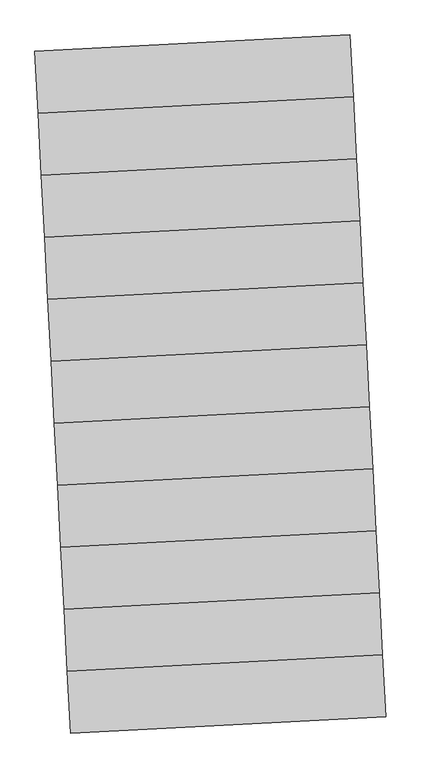
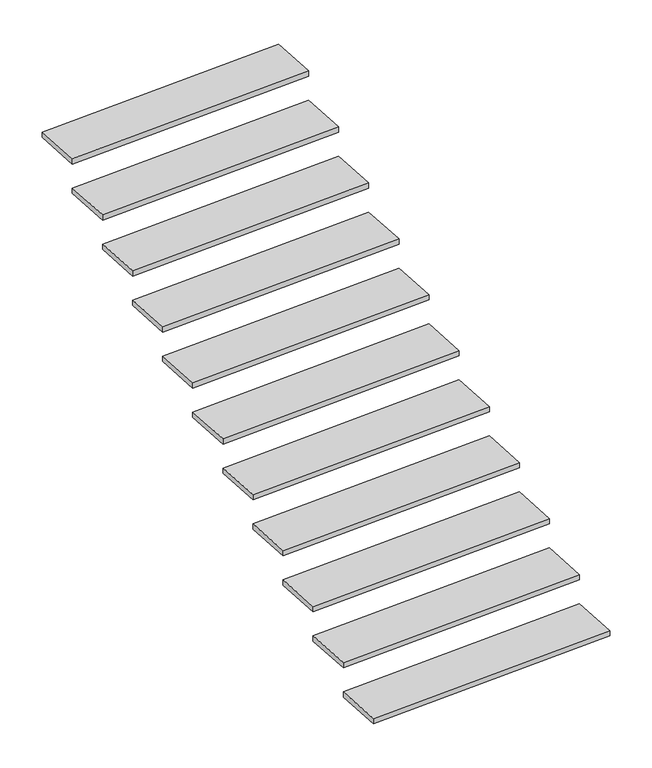
"""IFC4 building model written with IfcOpenShell, lengths in millimetres: stair flight geometry."""

import ifcopenshell
import ifcopenshell.guid

model = None  # the IFC model being written
_history = None  # IfcOwnerHistory: only IFC2X3 demands one
_inside = {}  # id of a spatial element -> (the spatial element, [elements in it])
_under = {}  # id of a project, library or spatial element -> (it, [spatial elements below it])
_declared = {}  # id of a project -> (the project, [libraries it declares])
_typed = {}  # id of a type object -> (the type object, [elements of that type])
_made_of = {}  # id of a material, layer set ... -> (it, [elements and type objects made of it])


def new_model(schema):
    """Start an empty IFC model of exactly this schema.

    Asked for "IFC4X3", IfcOpenShell would pick the latest addendum, in which some entities
    have other attributes; the version numbers below select the first issue.
    IFC2X3 requires an IfcOwnerHistory on every rooted entity: one is made here for all.
    """
    global model, _history
    if schema == "IFC4X3":
        model = ifcopenshell.file(schema_version=(4, 3, 0, 0))
    else:
        model = ifcopenshell.file(schema=schema)
    _inside.clear()
    _under.clear()
    _declared.clear()
    _typed.clear()
    _made_of.clear()
    _history = None
    if model.schema == "IFC2X3":
        org = make("IfcOrganization", Name="unknown")
        user = make(
            "IfcPersonAndOrganization",
            ThePerson=make("IfcPerson", FamilyName="unknown"),
            TheOrganization=org,
        )
        app = make(
            "IfcApplication",
            ApplicationDeveloper=org,
            Version="unknown",
            ApplicationFullName="unknown",
            ApplicationIdentifier="unknown",
        )
        _history = make(
            "IfcOwnerHistory",
            OwningUser=user,
            OwningApplication=app,
            ChangeAction="ADDED",
            CreationDate=0,
        )
    return model


def make(cls, **values):
    """One entity of the class cls with the attributes given. An attribute that is None is left unset."""
    return model.create_entity(
        cls, **{name: value for name, value in values.items() if value is not None}
    )


def rooted(cls, **values):
    """An entity with a GlobalId (a new one), such as an element, a storey or a relation."""
    return make(cls, GlobalId=ifcopenshell.guid.new(), OwnerHistory=_history, **values)


def si_unit(unit_type, name, prefix=None):
    """IfcSIUnit, for example si_unit("LENGTHUNIT", "METRE", prefix="MILLI")."""
    return make("IfcSIUnit", UnitType=unit_type, Prefix=prefix, Name=name)


def assignment(units):
    """IfcUnitAssignment: the units of a project."""
    return None if units is None else make("IfcUnitAssignment", Units=units)


def point(xyz):
    """IfcCartesianPoint."""
    return None if xyz is None else make("IfcCartesianPoint", Coordinates=xyz)


def direction(xyz):
    """IfcDirection."""
    return None if xyz is None else make("IfcDirection", DirectionRatios=xyz)


def frame(location, z_axis=None, x_axis=None):
    """IfcAxis2Placement3D, a coordinate frame: its origin and axes. An axis left out is left unset."""
    return make(
        "IfcAxis2Placement3D",
        Location=point(location),
        Axis=direction(z_axis),
        RefDirection=direction(x_axis),
    )


def origin():
    """The frame at (0, 0, 0) with its axes left unset."""
    return frame((0.0, 0.0, 0.0))


def place(relative_to, where):
    """IfcLocalPlacement: puts the frame where relative to a parent placement (None: the world)."""
    return make(
        "IfcLocalPlacement", PlacementRelTo=relative_to, RelativePlacement=where
    )


def context(
    kind, dimensions, precision=None, world=None, true_north=None, identifier=None
):
    """IfcGeometricRepresentationContext, for example the 3D "Model" context."""
    return make(
        "IfcGeometricRepresentationContext",
        ContextIdentifier=identifier,
        ContextType=kind,
        CoordinateSpaceDimension=dimensions,
        Precision=precision,
        WorldCoordinateSystem=world,
        TrueNorth=true_north,
    )


def project(units=None, contexts=None):
    """IfcProject with its units and contexts."""
    return rooted(
        "IfcProject",
        Name="project",
        RepresentationContexts=contexts,
        UnitsInContext=assignment(units),
    )


def spatial(cls, under=None, at=None, **own):
    """A site, building, storey or space (cls), placed at a placement, below another one or the project."""
    s = rooted(cls, ObjectPlacement=at, **own)
    if under is not None:
        _under.setdefault(under.id(), (under, []))[1].append(s)
    return s


def polyline(points):
    """IfcPolyline through the points."""
    return make("IfcPolyline", Points=[point(p) for p in points])


def outline(outer, holes=None, kind="AREA"):
    """IfcArbitraryClosedProfileDef: a profile drawn as a closed curve; with holes, ...WithVoids."""
    if holes is None:
        return make("IfcArbitraryClosedProfileDef", ProfileType=kind, OuterCurve=outer)
    return make(
        "IfcArbitraryProfileDefWithVoids",
        ProfileType=kind,
        OuterCurve=outer,
        InnerCurves=holes,
    )


def extrude(swept, where, along, depth):
    """IfcExtrudedAreaSolid: the profile swept, set in the frame where, extruded along a direction by depth."""
    return make(
        "IfcExtrudedAreaSolid",
        SweptArea=swept,
        Position=where,
        ExtrudedDirection=direction(along),
        Depth=depth,
    )


def shape(context_of_items, identifier, shape_type, items):
    """IfcShapeRepresentation: the items that make up one representation, for example the "Body"."""
    return make(
        "IfcShapeRepresentation",
        ContextOfItems=context_of_items,
        RepresentationIdentifier=identifier,
        RepresentationType=shape_type,
        Items=items,
    )


def source(mapping_origin, context_of_items, identifier, shape_type, items):
    """IfcRepresentationMap: a shape defined once, which mapped items show again and again."""
    return make(
        "IfcRepresentationMap",
        MappingOrigin=mapping_origin,
        MappedRepresentation=shape(context_of_items, identifier, shape_type, items),
    )


def transform(
    local_origin,
    x_axis=None,
    y_axis=None,
    z_axis=None,
    scale=None,
    scale2=None,
    scale3=None,
    uniform=True,
):
    """IfcCartesianTransformationOperator3D, or its non-uniform kind. x_axis, y_axis, z_axis: its Axis1, 2, 3."""
    if uniform:
        return make(
            "IfcCartesianTransformationOperator3D",
            Axis1=direction(x_axis),
            Axis2=direction(y_axis),
            LocalOrigin=point(local_origin),
            Scale=scale,
            Axis3=direction(z_axis),
        )
    return make(
        "IfcCartesianTransformationOperator3DnonUniform",
        Axis1=direction(x_axis),
        Axis2=direction(y_axis),
        LocalOrigin=point(local_origin),
        Scale=scale,
        Axis3=direction(z_axis),
        Scale2=scale2,
        Scale3=scale3,
    )


def mapped(mapping_source, mapping_target):
    """IfcMappedItem: shows the shape of a source again, moved by a transform."""
    return make(
        "IfcMappedItem", MappingSource=mapping_source, MappingTarget=mapping_target
    )


def made_of(thing, what):
    """Note that an element or type object is made of a material, layer set ...; save() writes the relation."""
    if what is not None:
        _made_of.setdefault(what.id(), (what, []))[1].append(thing)
    return thing


def element(
    cls,
    number,
    at=None,
    inside=None,
    cuts=None,
    type_object=None,
    material=None,
    context=None,
    identifier="Body",
    shape_type=None,
    held_by="IfcProductDefinitionShape",
    body=None,
    shapes=None,
    **own,
):
    """One element of the class cls, such as IfcWall. Its Tag is "e" and its number.

    at: its placement. inside: the storey or other place that contains it. cuts: it is an
    opening in that element (IfcRelVoidsElement). A single representation is given by context,
    identifier, shape_type and body (its items); several are given by shapes. held_by: the class
    of the entity that holds the representations. save() writes the other relations.
    """
    e = rooted(cls, Tag="e%d" % number, ObjectPlacement=at, **own)
    if body is not None:
        shapes = [shape(context, identifier, shape_type, body)]
    if shapes is not None:
        e.Representation = make(held_by, Representations=shapes)
    if inside is not None:
        _inside.setdefault(inside.id(), (inside, []))[1].append(e)
    if cuts is not None:
        rooted(
            "IfcRelVoidsElement", RelatingBuildingElement=cuts, RelatedOpeningElement=e
        )
    if type_object is not None:
        _typed.setdefault(type_object.id(), (type_object, []))[1].append(e)
    return made_of(e, material)


def aggregate(whole, parts):
    """IfcRelAggregates: a whole, such as a stair, and the parts it consists of."""
    return rooted("IfcRelAggregates", RelatingObject=whole, RelatedObjects=parts)


def save(model, path):
    """Write the relations noted so far, then the file.

    IfcRelAggregates (storeys below a building ...), IfcRelContainedInSpatialStructure (elements
    in a storey), IfcRelDefinesByType, IfcRelAssociatesMaterial and IfcRelDeclares: one each for
    every whole, place, type object, material and project.
    """
    for whole, parts in _under.values():
        aggregate(whole, parts)
    for where, things in _inside.values():
        rooted(
            "IfcRelContainedInSpatialStructure",
            RelatedElements=things,
            RelatingStructure=where,
        )
    for kind, things in _typed.values():
        rooted("IfcRelDefinesByType", RelatedObjects=things, RelatingType=kind)
    for what, things in _made_of.values():
        rooted("IfcRelAssociatesMaterial", RelatedObjects=things, RelatingMaterial=what)
    for by, libraries in _declared.values():
        rooted("IfcRelDeclares", RelatingContext=by, RelatedDefinitions=libraries)
    model.write(path)


def stair_flight_18440aeb(model_context):
    return source(origin(), model_context, "Body", "SweptSolid", [
        extrude(outline(polyline([(21524.3114867, 12733.1881413), (22897.427097, 12805.1500812), (22911.5578051, 12535.5201068), (21538.4421949, 12463.5581669), (21524.3114867, 12733.1881413)])), frame((0.0, 0.0, -157.0), z_axis=(0.0, 0.0, 1.0), x_axis=(1.0, 0.0, 0.0)), (0.0, 0.0, 1.0), 32.0),
        extrude(outline(polyline([(21510.1807785, 13002.8181157), (22883.2963888, 13074.7800555), (22897.427097, 12805.1500812), (21524.3114867, 12733.1881413), (21510.1807785, 13002.8181157)])), frame((0.0, 0.0, 18.0), z_axis=(0.0, 0.0, 1.0), x_axis=(1.0, 0.0, 0.0)), (0.0, 0.0, 1.0), 32.0),
        extrude(outline(polyline([(21496.0500703, 13272.4480901), (22869.1656806, 13344.4100299), (22883.2963888, 13074.7800555), (21510.1807785, 13002.8181157), (21496.0500703, 13272.4480901)])), frame((0.0, 0.0, 193.0), z_axis=(0.0, 0.0, 1.0), x_axis=(1.0, 0.0, 0.0)), (0.0, 0.0, 1.0), 32.0),
        extrude(outline(polyline([(21481.9193621, 13542.0780645), (22855.0349724, 13614.0400043), (22869.1656806, 13344.4100299), (21496.0500703, 13272.4480901), (21481.9193621, 13542.0780645)])), frame((0.0, 0.0, 368.0), z_axis=(0.0, 0.0, 1.0), x_axis=(1.0, 0.0, 0.0)), (0.0, 0.0, 1.0), 32.0),
        extrude(outline(polyline([(21467.7886539, 13811.7080389), (22840.9042642, 13883.6699787), (22855.0349724, 13614.0400043), (21481.9193621, 13542.0780645), (21467.7886539, 13811.7080389)])), frame((0.0, 0.0, 543.0), z_axis=(0.0, 0.0, 1.0), x_axis=(1.0, 0.0, 0.0)), (0.0, 0.0, 1.0), 32.0),
        extrude(outline(polyline([(21453.6579457, 14081.3380132), (22826.773556, 14153.2999531), (22840.9042642, 13883.6699787), (21467.7886539, 13811.7080389), (21453.6579457, 14081.3380132)])), frame((0.0, 0.0, 718.0), z_axis=(0.0, 0.0, 1.0), x_axis=(1.0, 0.0, 0.0)), (0.0, 0.0, 1.0), 32.0),
        extrude(outline(polyline([(21439.5272376, 14350.9679876), (22812.6428478, 14422.9299275), (22826.773556, 14153.2999531), (21453.6579457, 14081.3380132), (21439.5272376, 14350.9679876)])), frame((0.0, 0.0, 893.0), z_axis=(0.0, 0.0, 1.0), x_axis=(1.0, 0.0, 0.0)), (0.0, 0.0, 1.0), 32.0),
        extrude(outline(polyline([(21425.3965294, 14620.597962), (22798.5121397, 14692.5599018), (22812.6428478, 14422.9299275), (21439.5272376, 14350.9679876), (21425.3965294, 14620.597962)])), frame((0.0, 0.0, 1068.0), z_axis=(0.0, 0.0, 1.0), x_axis=(1.0, 0.0, 0.0)), (0.0, 0.0, 1.0), 32.0),
        extrude(outline(polyline([(21411.2658212, 14890.2279364), (22784.3814315, 14962.1898762), (22798.5121397, 14692.5599018), (21425.3965294, 14620.597962), (21411.2658212, 14890.2279364)])), frame((0.0, 0.0, 1243.0), z_axis=(0.0, 0.0, 1.0), x_axis=(1.0, 0.0, 0.0)), (0.0, 0.0, 1.0), 32.0),
        extrude(outline(polyline([(21397.135113, 15159.8579108), (22770.2507233, 15231.8198506), (22784.3814315, 14962.1898762), (21411.2658212, 14890.2279364), (21397.135113, 15159.8579108)])), frame((0.0, 0.0, 1418.0), z_axis=(0.0, 0.0, 1.0), x_axis=(1.0, 0.0, 0.0)), (0.0, 0.0, 1.0), 32.0),
        extrude(outline(polyline([(21383.0044048, 15429.4878852), (22756.1200151, 15501.449825), (22770.2507233, 15231.8198506), (21397.135113, 15159.8579108), (21383.0044048, 15429.4878852)])), frame((0.0, 0.0, 1593.0), z_axis=(0.0, 0.0, 1.0), x_axis=(1.0, 0.0, 0.0)), (0.0, 0.0, 1.0), 32.0),
    ])


if __name__ == "__main__":
    model = new_model("IFC4")
    model_context = context("Model", 3, world=origin())
    ifc_project = project(units=[si_unit("LENGTHUNIT", "METRE", prefix="MILLI")], contexts=[model_context])
    site = spatial("IfcSite", under=ifc_project)
    building = spatial("IfcBuilding", under=site)
    placement = place(None, origin())
    stair_flight_shape = stair_flight_18440aeb(model_context)
    element("IfcStairFlight", 1, at=placement, inside=building, context=model_context, shape_type="MappedRepresentation", body=[
        mapped(stair_flight_shape, transform((0.0, 0.0, 0.0), x_axis=(1.0, 0.0, 0.0), y_axis=(0.0, 1.0, 0.0), z_axis=(0.0, 0.0, 1.0))),
    ])
    save(model, "model.ifc")

# Revit data of these elements
# Project information
#   Building Name = "MAIN GATE SECURITY BUILDING"
#   Project Status = "Project Status"
#   Client Name = "현대엔지니어링"
#   Project Address = "서울시 종로구 율곡로 75(계동)"
#   Project Name = "Therma Visayas Energy Project"
#   Project Number = "-"
# Element 1 (IfcStairFlight)
#   Materials on its faces: "철강"
# Materials
#   "철강": class "Generic", colour RGB 143 142 141, transparency 0, Description = "철골+가공조립+세우기", Cost = 0
